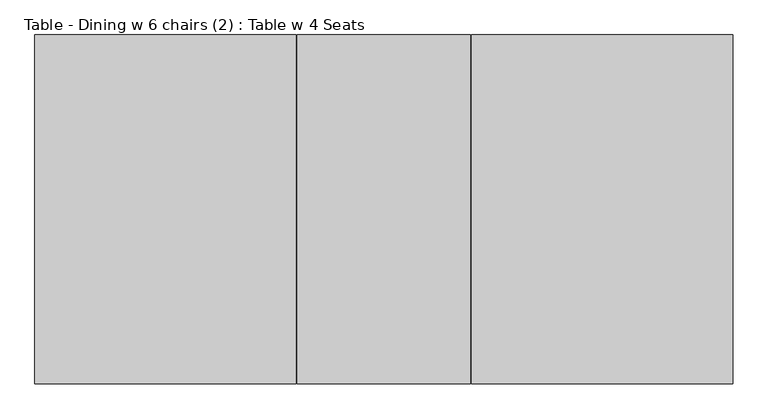
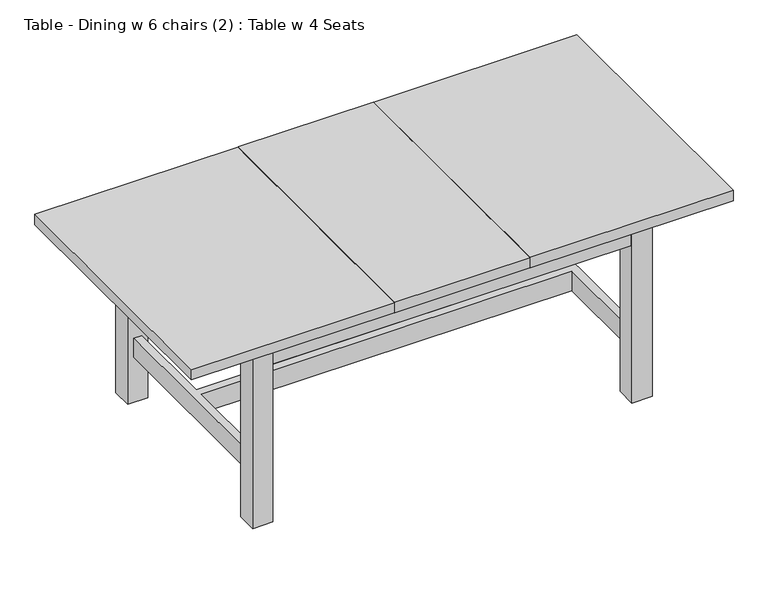
"""IFC4 building model written with IfcOpenShell, lengths in millimetres: furniture geometry, Table - Dining w 6 chairs (2) : Table w 4 Seats."""

import ifcopenshell
import ifcopenshell.guid

model = None  # the IFC model being written
_history = None  # IfcOwnerHistory: only IFC2X3 demands one
_inside = {}  # id of a spatial element -> (the spatial element, [elements in it])
_under = {}  # id of a project, library or spatial element -> (it, [spatial elements below it])
_declared = {}  # id of a project -> (the project, [libraries it declares])
_typed = {}  # id of a type object -> (the type object, [elements of that type])
_made_of = {}  # id of a material, layer set ... -> (it, [elements and type objects made of it])


def new_model(schema):
    """Start an empty IFC model of exactly this schema.

    Asked for "IFC4X3", IfcOpenShell would pick the latest addendum, in which some entities
    have other attributes; the version numbers below select the first issue.
    IFC2X3 requires an IfcOwnerHistory on every rooted entity: one is made here for all.
    """
    global model, _history
    if schema == "IFC4X3":
        model = ifcopenshell.file(schema_version=(4, 3, 0, 0))
    else:
        model = ifcopenshell.file(schema=schema)
    _inside.clear()
    _under.clear()
    _declared.clear()
    _typed.clear()
    _made_of.clear()
    _history = None
    if model.schema == "IFC2X3":
        org = make("IfcOrganization", Name="unknown")
        user = make(
            "IfcPersonAndOrganization",
            ThePerson=make("IfcPerson", FamilyName="unknown"),
            TheOrganization=org,
        )
        app = make(
            "IfcApplication",
            ApplicationDeveloper=org,
            Version="unknown",
            ApplicationFullName="unknown",
            ApplicationIdentifier="unknown",
        )
        _history = make(
            "IfcOwnerHistory",
            OwningUser=user,
            OwningApplication=app,
            ChangeAction="ADDED",
            CreationDate=0,
        )
    return model


def make(cls, **values):
    """One entity of the class cls with the attributes given. An attribute that is None is left unset."""
    return model.create_entity(
        cls, **{name: value for name, value in values.items() if value is not None}
    )


def rooted(cls, **values):
    """An entity with a GlobalId (a new one), such as an element, a storey or a relation."""
    return make(cls, GlobalId=ifcopenshell.guid.new(), OwnerHistory=_history, **values)


def si_unit(unit_type, name, prefix=None):
    """IfcSIUnit, for example si_unit("LENGTHUNIT", "METRE", prefix="MILLI")."""
    return make("IfcSIUnit", UnitType=unit_type, Prefix=prefix, Name=name)


def assignment(units):
    """IfcUnitAssignment: the units of a project."""
    return None if units is None else make("IfcUnitAssignment", Units=units)


def point(xyz):
    """IfcCartesianPoint."""
    return None if xyz is None else make("IfcCartesianPoint", Coordinates=xyz)


def direction(xyz):
    """IfcDirection."""
    return None if xyz is None else make("IfcDirection", DirectionRatios=xyz)


def frame(location, z_axis=None, x_axis=None):
    """IfcAxis2Placement3D, a coordinate frame: its origin and axes. An axis left out is left unset."""
    return make(
        "IfcAxis2Placement3D",
        Location=point(location),
        Axis=direction(z_axis),
        RefDirection=direction(x_axis),
    )


def origin():
    """The frame at (0, 0, 0) with its axes left unset."""
    return frame((0.0, 0.0, 0.0))


def origin_with_axes():
    """The frame at (0, 0, 0) with the z axis (0, 0, 1) and the x axis (1, 0, 0) written out."""
    return frame((0.0, 0.0, 0.0), z_axis=(0.0, 0.0, 1.0), x_axis=(1.0, 0.0, 0.0))


def place(relative_to, where):
    """IfcLocalPlacement: puts the frame where relative to a parent placement (None: the world)."""
    return make(
        "IfcLocalPlacement", PlacementRelTo=relative_to, RelativePlacement=where
    )


def context(
    kind, dimensions, precision=None, world=None, true_north=None, identifier=None
):
    """IfcGeometricRepresentationContext, for example the 3D "Model" context."""
    return make(
        "IfcGeometricRepresentationContext",
        ContextIdentifier=identifier,
        ContextType=kind,
        CoordinateSpaceDimension=dimensions,
        Precision=precision,
        WorldCoordinateSystem=world,
        TrueNorth=true_north,
    )


def project(units=None, contexts=None):
    """IfcProject with its units and contexts."""
    return rooted(
        "IfcProject",
        Name="project",
        RepresentationContexts=contexts,
        UnitsInContext=assignment(units),
    )


def spatial(cls, under=None, at=None, **own):
    """A site, building, storey or space (cls), placed at a placement, below another one or the project."""
    s = rooted(cls, ObjectPlacement=at, **own)
    if under is not None:
        _under.setdefault(under.id(), (under, []))[1].append(s)
    return s


def polyline(points):
    """IfcPolyline through the points."""
    return make("IfcPolyline", Points=[point(p) for p in points])


def outline(outer, holes=None, kind="AREA"):
    """IfcArbitraryClosedProfileDef: a profile drawn as a closed curve; with holes, ...WithVoids."""
    if holes is None:
        return make("IfcArbitraryClosedProfileDef", ProfileType=kind, OuterCurve=outer)
    return make(
        "IfcArbitraryProfileDefWithVoids",
        ProfileType=kind,
        OuterCurve=outer,
        InnerCurves=holes,
    )


def extrude(swept, where, along, depth):
    """IfcExtrudedAreaSolid: the profile swept, set in the frame where, extruded along a direction by depth."""
    return make(
        "IfcExtrudedAreaSolid",
        SweptArea=swept,
        Position=where,
        ExtrudedDirection=direction(along),
        Depth=depth,
    )


def faces_of(points, faces, orient=None, outer=None):
    """IfcFace entities. A face is a list of loops; a loop is a list of indices into points, from 0.

    orient and outer hold one flag for each loop. By default every Orientation is true, the
    first loop of a face is its IfcFaceOuterBound and the others are IfcFaceBound.
    """
    made = []
    for i, loops in enumerate(faces):
        bounds = []
        for j, loop in enumerate(loops):
            is_outer = j == 0 if outer is None else outer[i][j]
            bounds.append(
                make(
                    "IfcFaceOuterBound" if is_outer else "IfcFaceBound",
                    Bound=make("IfcPolyLoop", Polygon=[points[k] for k in loop]),
                    Orientation=True if orient is None else orient[i][j],
                )
            )
        made.append(make("IfcFace", Bounds=bounds))
    return made


def faceted_brep(points, faces, orient=None, outer=None, voids=None):
    """IfcFacetedBrep: a solid bounded by flat faces; with voids (closed shells), ...WithVoids."""
    shared = [point(p) for p in points]
    hull = make("IfcClosedShell", CfsFaces=faces_of(shared, faces, orient, outer))
    if voids is None:
        return make("IfcFacetedBrep", Outer=hull)
    return make(
        "IfcFacetedBrepWithVoids",
        Outer=hull,
        Voids=[
            make(cls, CfsFaces=faces_of(shared, fs, o, b)) for cls, fs, o, b in voids
        ],
    )


def shape(context_of_items, identifier, shape_type, items):
    """IfcShapeRepresentation: the items that make up one representation, for example the "Body"."""
    return make(
        "IfcShapeRepresentation",
        ContextOfItems=context_of_items,
        RepresentationIdentifier=identifier,
        RepresentationType=shape_type,
        Items=items,
    )


def source(mapping_origin, context_of_items, identifier, shape_type, items):
    """IfcRepresentationMap: a shape defined once, which mapped items show again and again."""
    return make(
        "IfcRepresentationMap",
        MappingOrigin=mapping_origin,
        MappedRepresentation=shape(context_of_items, identifier, shape_type, items),
    )


def transform(
    local_origin,
    x_axis=None,
    y_axis=None,
    z_axis=None,
    scale=None,
    scale2=None,
    scale3=None,
    uniform=True,
):
    """IfcCartesianTransformationOperator3D, or its non-uniform kind. x_axis, y_axis, z_axis: its Axis1, 2, 3."""
    if uniform:
        return make(
            "IfcCartesianTransformationOperator3D",
            Axis1=direction(x_axis),
            Axis2=direction(y_axis),
            LocalOrigin=point(local_origin),
            Scale=scale,
            Axis3=direction(z_axis),
        )
    return make(
        "IfcCartesianTransformationOperator3DnonUniform",
        Axis1=direction(x_axis),
        Axis2=direction(y_axis),
        LocalOrigin=point(local_origin),
        Scale=scale,
        Axis3=direction(z_axis),
        Scale2=scale2,
        Scale3=scale3,
    )


def mapped(mapping_source, mapping_target):
    """IfcMappedItem: shows the shape of a source again, moved by a transform."""
    return make(
        "IfcMappedItem", MappingSource=mapping_source, MappingTarget=mapping_target
    )


def made_of(thing, what):
    """Note that an element or type object is made of a material, layer set ...; save() writes the relation."""
    if what is not None:
        _made_of.setdefault(what.id(), (what, []))[1].append(thing)
    return thing


def element(
    cls,
    number,
    at=None,
    inside=None,
    cuts=None,
    type_object=None,
    material=None,
    context=None,
    identifier="Body",
    shape_type=None,
    held_by="IfcProductDefinitionShape",
    body=None,
    shapes=None,
    **own,
):
    """One element of the class cls, such as IfcWall. Its Tag is "e" and its number.

    at: its placement. inside: the storey or other place that contains it. cuts: it is an
    opening in that element (IfcRelVoidsElement). A single representation is given by context,
    identifier, shape_type and body (its items); several are given by shapes. held_by: the class
    of the entity that holds the representations. save() writes the other relations.
    """
    e = rooted(cls, Tag="e%d" % number, ObjectPlacement=at, **own)
    if body is not None:
        shapes = [shape(context, identifier, shape_type, body)]
    if shapes is not None:
        e.Representation = make(held_by, Representations=shapes)
    if inside is not None:
        _inside.setdefault(inside.id(), (inside, []))[1].append(e)
    if cuts is not None:
        rooted(
            "IfcRelVoidsElement", RelatingBuildingElement=cuts, RelatedOpeningElement=e
        )
    if type_object is not None:
        _typed.setdefault(type_object.id(), (type_object, []))[1].append(e)
    return made_of(e, material)


def aggregate(whole, parts):
    """IfcRelAggregates: a whole, such as a stair, and the parts it consists of."""
    return rooted("IfcRelAggregates", RelatingObject=whole, RelatedObjects=parts)


def save(model, path):
    """Write the relations noted so far, then the file.

    IfcRelAggregates (storeys below a building ...), IfcRelContainedInSpatialStructure (elements
    in a storey), IfcRelDefinesByType, IfcRelAssociatesMaterial and IfcRelDeclares: one each for
    every whole, place, type object, material and project.
    """
    for whole, parts in _under.values():
        aggregate(whole, parts)
    for where, things in _inside.values():
        rooted(
            "IfcRelContainedInSpatialStructure",
            RelatedElements=things,
            RelatingStructure=where,
        )
    for kind, things in _typed.values():
        rooted("IfcRelDefinesByType", RelatedObjects=things, RelatingType=kind)
    for what, things in _made_of.values():
        rooted("IfcRelAssociatesMaterial", RelatedObjects=things, RelatingMaterial=what)
    for by, libraries in _declared.values():
        rooted("IfcRelDeclares", RelatingContext=by, RelatedDefinitions=libraries)
    model.write(path)


def table_dining_w_6_chairs_2_table_w_4_seats_080c21d9(model_context):
    return source(origin(), model_context, "Body", "SolidModel", [
        extrude(outline(polyline([(-544.3212781, 474.3546292), (780.6787219, 474.3546292), (780.6787219, 454.3546292), (-544.3212781, 454.3546292), (-544.3212781, 474.3546292)])), frame((0.0, 0.0, 610.0), z_axis=(0.0, 0.0, 1.0), x_axis=(1.0, 0.0, 0.0)), (0.0, 0.0, 1.0), 100.0),
        extrude(outline(polyline([(-611.8212781, -318.1453708), (-611.8212781, 406.8546292), (-591.8212781, 406.8546292), (-591.8212781, -318.1453708), (-611.8212781, -318.1453708)])), frame((0.0, 0.0, 610.0), z_axis=(0.0, 0.0, 1.0), x_axis=(1.0, 0.0, 0.0)), (0.0, 0.0, 1.0), 100.0),
        extrude(outline(polyline([(780.6787219, -385.6453708), (-544.3212781, -385.6453708), (-544.3212781, -365.6453708), (780.6787219, -365.6453708), (780.6787219, -385.6453708)])), frame((0.0, 0.0, 610.0), z_axis=(0.0, 0.0, 1.0), x_axis=(1.0, 0.0, 0.0)), (0.0, 0.0, 1.0), 100.0),
        extrude(outline(polyline([(848.1787219, 406.8546292), (848.1787219, -318.1453708), (828.1787219, -318.1453708), (828.1787219, 406.8546292), (848.1787219, 406.8546292)])), frame((0.0, 0.0, 610.0), z_axis=(0.0, 0.0, 1.0), x_axis=(1.0, 0.0, 0.0)), (0.0, 0.0, 1.0), 100.0),
        extrude(outline(polyline([(-566.8212781, -318.1453708), (-596.8212781, -318.1453708), (-596.8212781, 406.8546292), (-566.8212781, 406.8546292), (-566.8212781, 59.3546292), (803.1787219, 59.3546292), (803.1787219, 406.8546292), (833.1787219, 406.8546292), (833.1787219, -318.1453708), (803.1787219, -318.1453708), (803.1787219, 29.3546292), (-566.8212781, 29.3546292), (-566.8212781, -318.1453708)])), frame((0.0, 0.0, 175.0), z_axis=(0.0, 0.0, 1.0), x_axis=(1.0, 0.0, 0.0)), (0.0, 0.0, 1.0), 75.0),
        extrude(outline(polyline([(-544.3212781, -393.1453708), (-619.3212781, -393.1453708), (-619.3212781, -318.1453708), (-544.3212781, -318.1453708), (-544.3212781, -393.1453708)])), origin_with_axes(), (0.0, 0.0, 1.0), 710.0),
        extrude(outline(polyline([(780.6787219, 481.8546292), (855.6787219, 481.8546292), (855.6787219, 406.8546292), (780.6787219, 406.8546292), (780.6787219, 481.8546292)])), origin_with_axes(), (0.0, 0.0, 1.0), 710.0),
        extrude(outline(polyline([(780.6787219, -318.1453708), (855.6787219, -318.1453708), (855.6787219, -393.1453708), (780.6787219, -393.1453708), (780.6787219, -318.1453708)])), origin_with_axes(), (0.0, 0.0, 1.0), 710.0),
        extrude(outline(polyline([(-544.3212781, 481.8546292), (-544.3212781, 406.8546292), (-619.3212781, 406.8546292), (-619.3212781, 481.8546292), (-544.3212781, 481.8546292)])), origin_with_axes(), (0.0, 0.0, 1.0), 710.0),
        faceted_brep([(1118.1787219, -455.6453708, 750.0), (1118.1787219, 544.3546292, 750.0), (369.6787219, 544.3546292, 750.0), (369.6787219, -455.6453708, 750.0), (-881.8212781, 544.3546292, 750.0), (-881.8212781, -455.6453708, 750.0), (-133.3212781, -455.6453708, 750.0), (-133.3212781, 544.3546292, 750.0), (366.6787219, 544.3546292, 750.0), (-130.3212781, 544.3546292, 750.0), (-130.3212781, -455.6453708, 750.0), (366.6787219, -455.6453708, 750.0), (-881.8212781, -455.6453708, 710.0), (-881.8212781, 544.3546292, 710.0), (-133.3212781, 544.3546292, 710.0), (-131.8212781, 542.8546292, 710.0), (-130.3212781, 544.3546292, 710.0), (366.6787219, 544.3546292, 710.0), (368.1787219, 542.8546292, 710.0), (369.6787219, 544.3546292, 710.0), (1118.1787219, 544.3546292, 710.0), (1118.1787219, -455.6453708, 710.0), (369.6787219, -455.6453708, 710.0), (368.1787219, -454.1453708, 710.0), (366.6787219, -455.6453708, 710.0), (-130.3212781, -455.6453708, 710.0), (-131.8212781, -454.1453708, 710.0), (-133.3212781, -455.6453708, 710.0), (-131.8212781, 542.8546292, 748.5), (368.1787219, 542.8546292, 748.5), (-131.8212781, -454.1453708, 748.5), (368.1787219, -454.1453708, 748.5)], [[[0, 1, 2, 3]], [[4, 5, 6, 7]], [[8, 9, 10, 11]], [[12, 13, 14, 15, 16, 17, 18, 19, 20, 21, 22, 23, 24, 25, 26, 27]], [[1, 0, 21, 20]], [[9, 8, 17, 16]], [[1, 20, 19, 2]], [[13, 4, 7, 14]], [[5, 4, 13, 12]], [[11, 10, 25, 24]], [[21, 0, 3, 22]], [[5, 12, 27, 6]], [[15, 28, 9, 16]], [[28, 15, 14, 7]], [[18, 29, 2, 19]], [[29, 18, 17, 8]], [[9, 28, 30, 10]], [[28, 7, 6, 30]], [[2, 29, 31, 3]], [[29, 8, 11, 31]], [[10, 30, 26, 25]], [[30, 6, 27, 26]], [[3, 31, 23, 22]], [[31, 11, 24, 23]]]),
    ])


if __name__ == "__main__":
    model = new_model("IFC4")
    model_context = context("Model", 3, world=origin())
    ifc_project = project(units=[si_unit("LENGTHUNIT", "METRE", prefix="MILLI")], contexts=[model_context])
    site = spatial("IfcSite", under=ifc_project)
    building = spatial("IfcBuilding", under=site)
    placement = place(None, origin())
    table_dining_w_6_chairs_2_table_w_4_seats_shape = table_dining_w_6_chairs_2_table_w_4_seats_080c21d9(model_context)
    element("IfcFurniture", 1, ObjectType="Table - Dining w 6 chairs (2) : Table w 4 Seats", at=placement, inside=building, context=model_context, shape_type="MappedRepresentation", body=[
        mapped(table_dining_w_6_chairs_2_table_w_4_seats_shape, transform((0.0, 0.0, 0.0), x_axis=(1.0, 0.0, 0.0), y_axis=(0.0, 1.0, 0.0), z_axis=(0.0, 0.0, 1.0))),
    ])
    save(model, "model.ifc")

# Revit data of these elements
# Project information
#   Project Status = "Project Status"
#   Client Name = "Revit Project"
#   Project Address = "Enter address here"
#   Project Name = "Two Storey Residence"
#   Project Number = "P.01"
# Type "Table - Dining w 6 chairs (2) : Table w 4 Seats"
#   Keynote = "N"
#   Width = 1000 mm
#   Table Top Thickness = 40 mm
#   Table Height = 750 mm
#   Length = 2000 mm
#   Leg Width = 75 mm
#   Leg Spacing Width = 800 mm
#   Leg Spacing Length = 1400 mm
#   Chair Side Spacing = 700 mm
#   Centre Piece = 500 mm
#   Vis - End Chairs = no
#   Material Table = Wood - Birch
#   Material Chair Structure = Wood - Birch
#   Material Chair Covering = Fabric - Beige
#   Default Elevation = 0
# Element 1 (IfcFurniture, "Table - Dining w 6 chairs (2) : Table w 4 Seats")
#   Materials on its faces: "Wood - Birch"
# Materials
#   "Wood - Birch": class "Wood", colour RGB 224 178 126, transparency 0
#   "Fabric - Beige": class "Fabric", colour RGB 231 227 195, transparency 0
